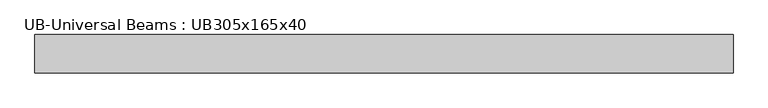
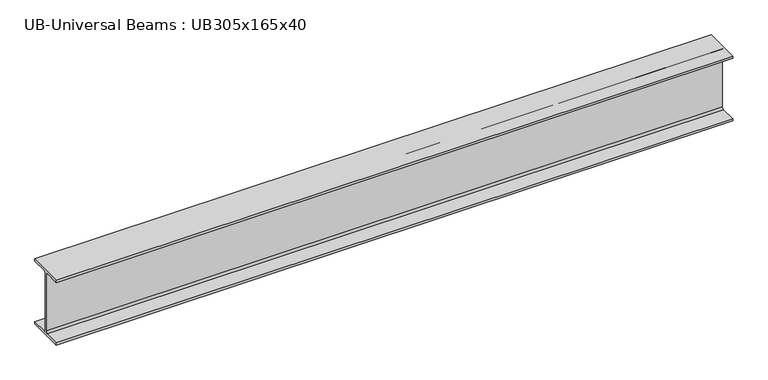
"""IFC4 building model written with IfcOpenShell, lengths in millimetres: beam geometry, UB-Universal Beams : UB305x165x40."""

from ifc_helpers import new_model, si_unit, point, frame, frame_2d, origin, place, context, project, spatial, polyline, circle_curve, trimmed, segment, composite_curve, outline, extrude, source, transform, mapped, element, save


def ub_universal_beams_ub305x165x40_8b2c45c1(model_context):
    return source(origin(), model_context, "Body", "SweptSolid", [
        extrude(outline(composite_curve([segment(polyline([(82.5, -141.5), (82.5, -151.7), (-82.5, -151.7), (-82.5, -141.5), (-11.9, -141.5)]), True, "CONTINUOUS"), segment(trimmed(circle_curve(frame_2d((-11.9, -132.6)), 8.9), [point((-11.9, -141.5))], [point((-3.0, -132.6))], True, "CARTESIAN"), True, "CONTINUOUS"), segment(polyline([(-3.0, -132.6), (-3.0, 132.6)]), True, "CONTINUOUS"), segment(trimmed(circle_curve(frame_2d((-11.9, 132.6)), 8.9), [point((-3.0, 132.6))], [point((-11.9, 141.5))], True, "CARTESIAN"), True, "CONTINUOUS"), segment(polyline([(-11.9, 141.5), (-82.5, 141.5), (-82.5, 151.7), (82.5, 151.7), (82.5, 141.5), (11.9, 141.5)]), True, "CONTINUOUS"), segment(trimmed(circle_curve(frame_2d((11.9, 132.6)), 8.9), [point((11.9, 141.5))], [point((3.0, 132.6))], True, "CARTESIAN"), True, "CONTINUOUS"), segment(polyline([(3.0, 132.6), (3.0, -132.6)]), True, "CONTINUOUS"), segment(trimmed(circle_curve(frame_2d((11.9, -132.6)), 8.9), [point((3.0, -132.6))], [point((11.9, -141.5))], True, "CARTESIAN"), True, "CONTINUOUS"), segment(polyline([(11.9, -141.5), (82.5, -141.5)]), True, "CONTINUOUS")], self_intersect=False)), frame((-1500.0, 0.0, 0.0), z_axis=(1.0, 0.0, 0.0), x_axis=(0.0, 1.0, 0.0)), (0.0, 0.0, 1.0), 3000.0),
    ])


if __name__ == "__main__":
    model = new_model("IFC4")
    model_context = context("Model", 3, world=origin())
    ifc_project = project(units=[si_unit("LENGTHUNIT", "METRE", prefix="MILLI")], contexts=[model_context])
    site = spatial("IfcSite", under=ifc_project)
    building = spatial("IfcBuilding", under=site)
    placement = place(None, origin())
    ub_universal_beams_ub305x165x40_shape = ub_universal_beams_ub305x165x40_8b2c45c1(model_context)
    element("IfcBeam", 1, ObjectType="UB-Universal Beams : UB305x165x40", at=placement, inside=building, context=model_context, shape_type="MappedRepresentation", body=[
        mapped(ub_universal_beams_ub305x165x40_shape, transform((0.0, 0.0, 0.0), x_axis=(1.0, 0.0, 0.0), y_axis=(0.0, 1.0, 0.0), z_axis=(0.0, 0.0, 1.0))),
    ])
    save(model, "model.ifc")

# Revit data of these elements
# Type "UB-Universal Beams : UB305x165x40"
#   Section Name Key = "UB305X165X40"
#   Width = 16.5 cm
#   Web Thickness = 0.6 cm
#   Web Fillet = 0.89 cm
#   Warping Constant = 164000.0 cm⁶
#   Torsional Moment of Inertia = 14.70 cm⁴
#   Section Area = 51.3 cm²
#   Plastic Modulus weak axis = 142.0 cm³
#   Plastic Modulus strong axis = 623.0 cm³
#   Nominal Weight = 40.2999 kgf/m
#   Moment of Inertia weak axis = 764.00 cm⁴
#   Moment of Inertia strong axis = 8503.00 cm⁴
#   Height = 30.34 cm
#   Flange Thickness = 1.02 cm
#   Elastic Modulus weak axis = 92.6 cm³
#   Elastic Modulus strong axis = 560.0 cm³
#   Centroid Vertical = 15.17 cm
#   Centroid Horizontal = 8.25 cm
#   Bolt Spacing = 9.0 cm
#   Length [instance default] = 1500 mm
#   Structural Material [instance default] = Metal - Steel 43-275
#   Type Comments = ""
#   Assembly Code = ""
# Element 1 (IfcBeam, "UB-Universal Beams : UB305x165x40")
#   Materials on its faces: "Metal - Steel 43-275"
# Materials
#   "Metal - Steel 43-275": class "Metal", colour RGB 247 247 247, transparency 0, Cost = 0
